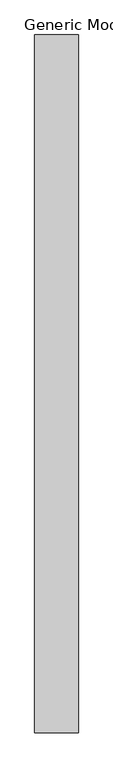
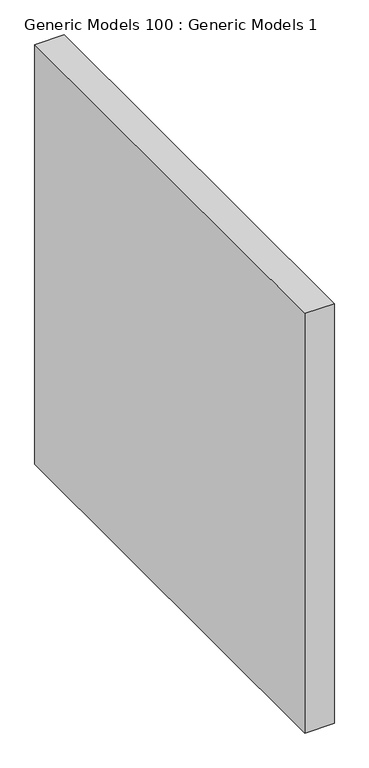
"""IFC4 building model written with IfcOpenShell, lengths in millimetres: proxy geometry, Generic Models 100 : Generic Models 1."""

from ifc_helpers import new_model, si_unit, frame, origin, place, context, project, spatial, polyline, outline, extrude, source, transform, mapped, element, save


def generic_models_100_generic_models_1_fed90478(model_context):
    return source(origin(), model_context, "Body", "SweptSolid", [
        extrude(outline(polyline([(52216.05, 1219.2), (52216.05, 0.0), (52139.85, 0.0), (52139.85, 1219.2), (52216.05, 1219.2)])), frame((0.0, 0.0, 3211.5125), z_axis=(0.0, 0.0, 1.0), x_axis=(1.0, 0.0, 0.0)), (0.0, 0.0, 1.0), 1155.7),
    ])


if __name__ == "__main__":
    model = new_model("IFC4")
    model_context = context("Model", 3, world=origin())
    ifc_project = project(units=[si_unit("LENGTHUNIT", "METRE", prefix="MILLI")], contexts=[model_context])
    site = spatial("IfcSite", under=ifc_project)
    building = spatial("IfcBuilding", under=site)
    placement = place(None, origin())
    generic_models_100_generic_models_1_shape = generic_models_100_generic_models_1_fed90478(model_context)
    element("IfcBuildingElementProxy", 1, Name="Generic Models 100 : Generic Models 1", ObjectType="Generic Models 100 : Generic Models 1", at=placement, inside=building, context=model_context, shape_type="MappedRepresentation", body=[
        mapped(generic_models_100_generic_models_1_shape, transform((0.0, 0.0, 0.0), x_axis=(1.0, 0.0, 0.0), y_axis=(0.0, 1.0, 0.0), z_axis=(0.0, 0.0, 1.0))),
    ])
    save(model, "model.ifc")

# Revit data of these elements
# Element 1 (IfcBuildingElementProxy, "Generic Models 100 : Generic Models 1")
#   Materials on its faces: "(S) SOUND BATT. INSULATION (THICKNESS TO MATCH WALL DEPTH)"
# Materials
#   "(S) SOUND BATT. INSULATION (THICKNESS TO MATCH WALL DEPTH)": class "Unassigned", colour RGB 255 255 255, transparency 0, Cost = 0
